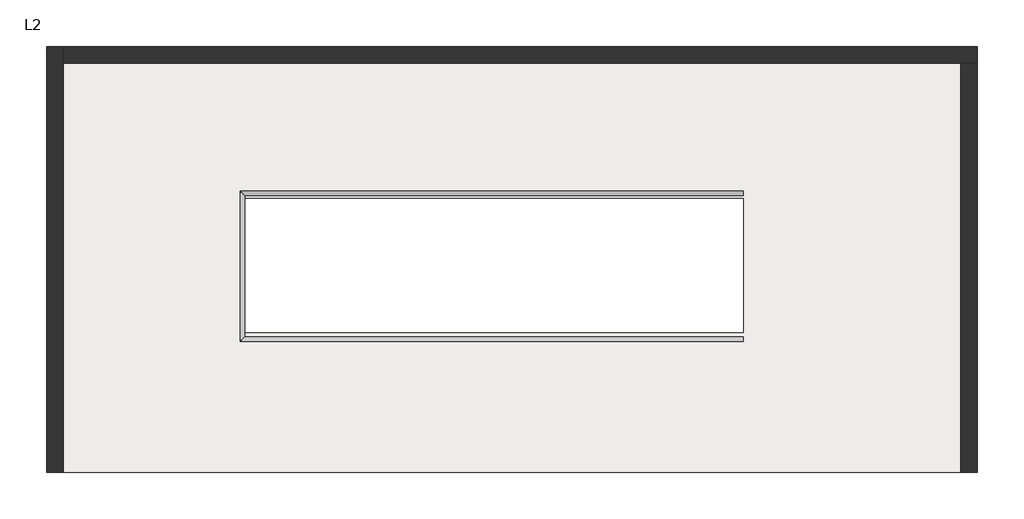
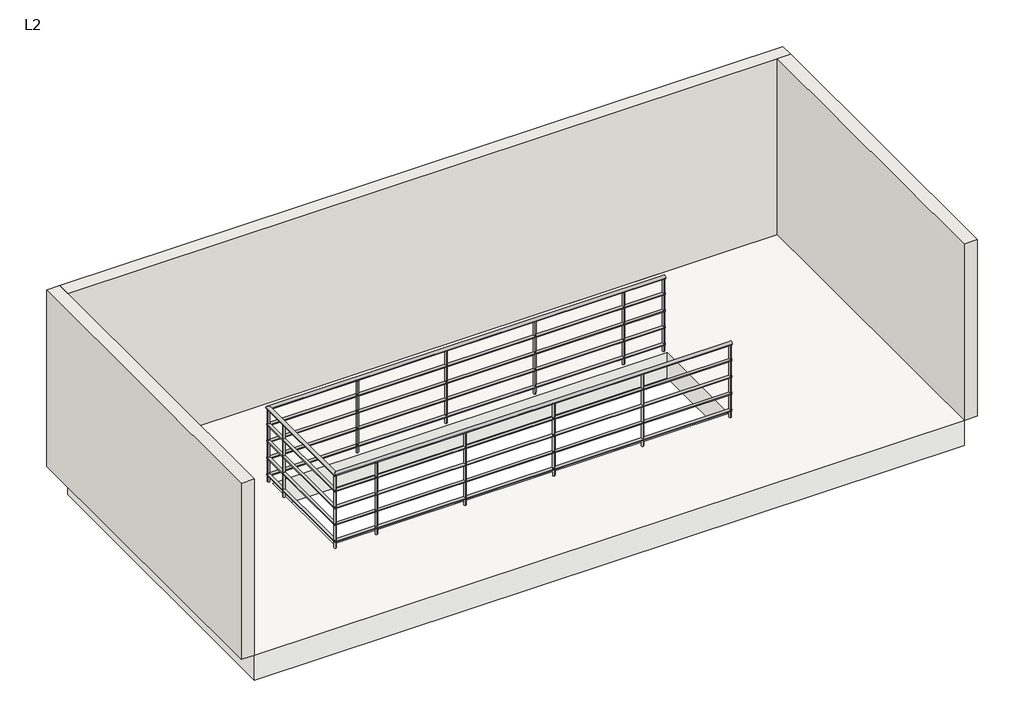
# One storey: 3 walls, 1 railing, 1 slab.
"""IFC4 building model written with IfcOpenShell, lengths in millimetres."""

from ifc_helpers import new_model, si_unit, point, frame, frame_2d, origin, place, context, project, spatial, polyline, circle_curve, ellipse_curve, trimmed, segment, composite_curve, outline, extrude, faceted_brep, element, save
from ifc_brep_helpers import plane_surface, cylinder_surface, advanced_brep

model = new_model("IFC4")

# Units and contexts
model_context = context("Model", 3, world=origin())
ifc_project = project(units=[si_unit("LENGTHUNIT", "METRE", prefix="MILLI")], contexts=[model_context])

# Site, building, storey
site = spatial("IfcSite", under=ifc_project)
building = spatial("IfcBuilding", under=site)
storey = spatial("IfcBuildingStorey", under=building, Name="L2", Elevation=2700.0)

# Railing
placement = place(None, origin())
element("IfcRailing", 1, ObjectType="900mm Pipe", at=placement, inside=storey, context=model_context, shape_type="SolidModel", body=[
    advanced_brep(
    [(-2164.8480531, 1633.4805305, 3580.0), (-2164.8480531, 1593.4805305, 3580.0), (-6608.8480531, 1633.4805305, 3580.0), (-6648.8480531, 1593.4805305, 3580.0), (-6608.8480531, 2893.4805305, 3580.0), (-6648.8480531, 2933.4805305, 3580.0), (-2164.8480531, 2893.4805305, 3580.0), (-2164.8480531, 2933.4805305, 3580.0)],
    [
        (0, 1, circle_curve(frame((-2164.8480531, 1613.4805305, 3580.0), z_axis=(1.0, 0.0, 0.0), x_axis=(0.0, -1.0, 0.0)), 20.0)),
        (1, 0, circle_curve(frame((-2164.8480531, 1613.4805305, 3580.0), z_axis=(1.0, 0.0, 0.0), x_axis=(0.0, -1.0, 0.0)), 20.0)),
        (0, 2),
        (2, 3, ellipse_curve(frame((-6628.8480531, 1613.4805305, 3580.0), z_axis=(0.7071067811865459, -0.7071067811865491, 0.0), x_axis=(0.7071067811865491, 0.7071067811865459, 0.0)), 28.2842712, 20.0)),
        (3, 1),
        (3, 2, ellipse_curve(frame((-6628.8480531, 1613.4805305, 3580.0), z_axis=(0.7071067811865459, -0.7071067811865491, 0.0), x_axis=(0.7071067811865491, 0.7071067811865459, 0.0)), 28.2842712, 20.0)),
        (2, 4),
        (4, 5, ellipse_curve(frame((-6628.8480531, 2913.4805305, 3580.0), z_axis=(-0.7071067811865492, -0.7071067811865458, 0.0), x_axis=(0.7071067811865457, -0.7071067811865493, 0.0)), 28.2842712, 20.0)),
        (5, 3),
        (5, 4, ellipse_curve(frame((-6628.8480531, 2913.4805305, 3580.0), z_axis=(-0.7071067811865492, -0.7071067811865458, 0.0), x_axis=(0.7071067811865457, -0.7071067811865493, 0.0)), 28.2842712, 20.0)),
        (6, 7, circle_curve(frame((-2164.8480531, 2913.4805305, 3580.0), z_axis=(1.0, 0.0, 0.0), x_axis=(0.0, 1.0, 0.0)), 20.0)),
        (7, 6, circle_curve(frame((-2164.8480531, 2913.4805305, 3580.0), z_axis=(1.0, 0.0, 0.0), x_axis=(0.0, 1.0, 0.0)), 20.0)),
        (4, 6),
        (7, 5),
    ],
    [
        plane_surface(frame((-2164.8480531, 1613.4805305, 3600.0), z_axis=(1.0, 0.0, 0.0), x_axis=(0.0, -1.0, 0.0))),
        cylinder_surface(frame((-2164.8480531, 1613.4805305, 3580.0), z_axis=(1.0, 0.0, 0.0), x_axis=(0.0, -1.0, 0.0)), 20.0),
        cylinder_surface(frame((-6628.8480531, 1613.4805305, 3580.0), z_axis=(0.0, -1.0, 0.0), x_axis=(-1.0, 0.0, 0.0)), 20.0),
        plane_surface(frame((-2164.8480531, 2913.4805305, 3600.0), z_axis=(1.0, 0.0, 0.0), x_axis=(0.0, 1.0, 0.0))),
        cylinder_surface(frame((-6628.8480531, 2913.4805305, 3580.0), z_axis=(-1.0, 0.0, 0.0), x_axis=(0.0, 1.0, 0.0)), 20.0),
    ],
    [
        (0, [[1, 2]]),
        (1, [[-1, 3, 4, 5]]),
        (1, [[-2, -5, 6, -3]]),
        (2, [[-4, 7, 8, 9]]),
        (2, [[-6, -9, 10, -7]]),
        (3, [[11, 12]]),
        (4, [[-8, 13, -12, 14]]),
        (4, [[-10, -14, -11, -13]]),
    ],
),
    advanced_brep(
    [(-2164.8480531, 1598.4805305, 3385.0), (-2164.8480531, 1628.4805305, 3385.0), (-6643.8480531, 1598.4805305, 3385.0), (-6613.8480531, 1628.4805305, 3385.0), (-6643.8480531, 2928.4805305, 3385.0), (-6613.8480531, 2898.4805305, 3385.0), (-2164.8480531, 2928.4805305, 3385.0), (-2164.8480531, 2898.4805305, 3385.0)],
    [
        (0, 1, circle_curve(frame((-2164.8480531, 1613.4805305, 3385.0), z_axis=(1.0, 0.0, 0.0), x_axis=(0.0, 1.0, 0.0)), 15.0)),
        (1, 0, circle_curve(frame((-2164.8480531, 1613.4805305, 3385.0), z_axis=(1.0, 0.0, 0.0), x_axis=(0.0, 1.0, 0.0)), 15.0)),
        (0, 2),
        (2, 3, ellipse_curve(frame((-6628.8480531, 1613.4805305, 3385.0), z_axis=(0.7071067811865459, -0.7071067811865491, 0.0), x_axis=(0.7071067811865491, 0.7071067811865459, 0.0)), 21.2132034, 15.0)),
        (3, 1),
        (3, 2, ellipse_curve(frame((-6628.8480531, 1613.4805305, 3385.0), z_axis=(0.7071067811865459, -0.7071067811865491, 0.0), x_axis=(0.7071067811865491, 0.7071067811865459, 0.0)), 21.2132034, 15.0)),
        (2, 4),
        (4, 5, ellipse_curve(frame((-6628.8480531, 2913.4805305, 3385.0), z_axis=(-0.7071067811865492, -0.7071067811865458, 0.0), x_axis=(0.7071067811865457, -0.7071067811865493, 0.0)), 21.2132034, 15.0)),
        (5, 3),
        (5, 4, ellipse_curve(frame((-6628.8480531, 2913.4805305, 3385.0), z_axis=(-0.7071067811865492, -0.7071067811865458, 0.0), x_axis=(0.7071067811865457, -0.7071067811865493, 0.0)), 21.2132034, 15.0)),
        (6, 7, circle_curve(frame((-2164.8480531, 2913.4805305, 3385.0), z_axis=(1.0, 0.0, 0.0), x_axis=(0.0, -1.0, 0.0)), 15.0)),
        (7, 6, circle_curve(frame((-2164.8480531, 2913.4805305, 3385.0), z_axis=(1.0, 0.0, 0.0), x_axis=(0.0, -1.0, 0.0)), 15.0)),
        (4, 6),
        (7, 5),
    ],
    [
        plane_surface(frame((-2164.8480531, 1613.4805305, 3400.0), z_axis=(1.0, 0.0, 0.0), x_axis=(0.0, -1.0, 0.0))),
        cylinder_surface(frame((-2164.8480531, 1613.4805305, 3385.0), z_axis=(1.0, 0.0, 0.0), x_axis=(0.0, 1.0, 0.0)), 15.0),
        cylinder_surface(frame((-6628.8480531, 1613.4805305, 3385.0), z_axis=(0.0, -1.0, 0.0), x_axis=(1.0, 0.0, 0.0)), 15.0),
        plane_surface(frame((-2164.8480531, 2913.4805305, 3400.0), z_axis=(1.0, 0.0, 0.0), x_axis=(0.0, 1.0, 0.0))),
        cylinder_surface(frame((-6628.8480531, 2913.4805305, 3385.0), z_axis=(-1.0, 0.0, 0.0), x_axis=(0.0, -1.0, 0.0)), 15.0),
    ],
    [
        (0, [[1, 2]]),
        (1, [[-1, 3, 4, 5]]),
        (1, [[-2, -5, 6, -3]]),
        (2, [[-4, 7, 8, 9]]),
        (2, [[-6, -9, 10, -7]]),
        (3, [[11, 12]]),
        (4, [[-8, 13, -12, 14]]),
        (4, [[-10, -14, -11, -13]]),
    ],
),
    advanced_brep(
    [(-2164.8480531, 1598.4805305, 3185.0), (-2164.8480531, 1628.4805305, 3185.0), (-6643.8480531, 1598.4805305, 3185.0), (-6613.8480531, 1628.4805305, 3185.0), (-6643.8480531, 2928.4805305, 3185.0), (-6613.8480531, 2898.4805305, 3185.0), (-2164.8480531, 2928.4805305, 3185.0), (-2164.8480531, 2898.4805305, 3185.0)],
    [
        (0, 1, circle_curve(frame((-2164.8480531, 1613.4805305, 3185.0), z_axis=(1.0, 0.0, 0.0), x_axis=(0.0, 1.0, 0.0)), 15.0)),
        (1, 0, circle_curve(frame((-2164.8480531, 1613.4805305, 3185.0), z_axis=(1.0, 0.0, 0.0), x_axis=(0.0, 1.0, 0.0)), 15.0)),
        (0, 2),
        (2, 3, ellipse_curve(frame((-6628.8480531, 1613.4805305, 3185.0), z_axis=(0.7071067811865459, -0.7071067811865491, 0.0), x_axis=(0.7071067811865491, 0.7071067811865459, 0.0)), 21.2132034, 15.0)),
        (3, 1),
        (3, 2, ellipse_curve(frame((-6628.8480531, 1613.4805305, 3185.0), z_axis=(0.7071067811865459, -0.7071067811865491, 0.0), x_axis=(0.7071067811865491, 0.7071067811865459, 0.0)), 21.2132034, 15.0)),
        (2, 4),
        (4, 5, ellipse_curve(frame((-6628.8480531, 2913.4805305, 3185.0), z_axis=(-0.7071067811865492, -0.7071067811865458, 0.0), x_axis=(0.7071067811865457, -0.7071067811865493, 0.0)), 21.2132034, 15.0)),
        (5, 3),
        (5, 4, ellipse_curve(frame((-6628.8480531, 2913.4805305, 3185.0), z_axis=(-0.7071067811865492, -0.7071067811865458, 0.0), x_axis=(0.7071067811865457, -0.7071067811865493, 0.0)), 21.2132034, 15.0)),
        (6, 7, circle_curve(frame((-2164.8480531, 2913.4805305, 3185.0), z_axis=(1.0, 0.0, 0.0), x_axis=(0.0, -1.0, 0.0)), 15.0)),
        (7, 6, circle_curve(frame((-2164.8480531, 2913.4805305, 3185.0), z_axis=(1.0, 0.0, 0.0), x_axis=(0.0, -1.0, 0.0)), 15.0)),
        (4, 6),
        (7, 5),
    ],
    [
        plane_surface(frame((-2164.8480531, 1613.4805305, 3200.0), z_axis=(1.0, 0.0, 0.0), x_axis=(0.0, -1.0, 0.0))),
        cylinder_surface(frame((-2164.8480531, 1613.4805305, 3185.0), z_axis=(1.0, 0.0, 0.0), x_axis=(0.0, 1.0, 0.0)), 15.0),
        cylinder_surface(frame((-6628.8480531, 1613.4805305, 3185.0), z_axis=(0.0, -1.0, 0.0), x_axis=(1.0, 0.0, 0.0)), 15.0),
        plane_surface(frame((-2164.8480531, 2913.4805305, 3200.0), z_axis=(1.0, 0.0, 0.0), x_axis=(0.0, 1.0, 0.0))),
        cylinder_surface(frame((-6628.8480531, 2913.4805305, 3185.0), z_axis=(-1.0, 0.0, 0.0), x_axis=(0.0, -1.0, 0.0)), 15.0),
    ],
    [
        (0, [[1, 2]]),
        (1, [[-1, 3, 4, 5]]),
        (1, [[-2, -5, 6, -3]]),
        (2, [[-4, 7, 8, 9]]),
        (2, [[-6, -9, 10, -7]]),
        (3, [[11, 12]]),
        (4, [[-8, 13, -12, 14]]),
        (4, [[-10, -14, -11, -13]]),
    ],
),
    advanced_brep(
    [(-2164.8480531, 1598.4805305, 2985.0), (-2164.8480531, 1628.4805305, 2985.0), (-6643.8480531, 1598.4805305, 2985.0), (-6613.8480531, 1628.4805305, 2985.0), (-6643.8480531, 2928.4805305, 2985.0), (-6613.8480531, 2898.4805305, 2985.0), (-2164.8480531, 2928.4805305, 2985.0), (-2164.8480531, 2898.4805305, 2985.0)],
    [
        (0, 1, circle_curve(frame((-2164.8480531, 1613.4805305, 2985.0), z_axis=(1.0, 0.0, 0.0), x_axis=(0.0, 1.0, 0.0)), 15.0)),
        (1, 0, circle_curve(frame((-2164.8480531, 1613.4805305, 2985.0), z_axis=(1.0, 0.0, 0.0), x_axis=(0.0, 1.0, 0.0)), 15.0)),
        (0, 2),
        (2, 3, ellipse_curve(frame((-6628.8480531, 1613.4805305, 2985.0), z_axis=(0.7071067811865459, -0.7071067811865491, 0.0), x_axis=(0.7071067811865491, 0.7071067811865459, 0.0)), 21.2132034, 15.0)),
        (3, 1),
        (3, 2, ellipse_curve(frame((-6628.8480531, 1613.4805305, 2985.0), z_axis=(0.7071067811865459, -0.7071067811865491, 0.0), x_axis=(0.7071067811865491, 0.7071067811865459, 0.0)), 21.2132034, 15.0)),
        (2, 4),
        (4, 5, ellipse_curve(frame((-6628.8480531, 2913.4805305, 2985.0), z_axis=(-0.7071067811865492, -0.7071067811865458, 0.0), x_axis=(0.7071067811865457, -0.7071067811865493, 0.0)), 21.2132034, 15.0)),
        (5, 3),
        (5, 4, ellipse_curve(frame((-6628.8480531, 2913.4805305, 2985.0), z_axis=(-0.7071067811865492, -0.7071067811865458, 0.0), x_axis=(0.7071067811865457, -0.7071067811865493, 0.0)), 21.2132034, 15.0)),
        (6, 7, circle_curve(frame((-2164.8480531, 2913.4805305, 2985.0), z_axis=(1.0, 0.0, 0.0), x_axis=(0.0, -1.0, 0.0)), 15.0)),
        (7, 6, circle_curve(frame((-2164.8480531, 2913.4805305, 2985.0), z_axis=(1.0, 0.0, 0.0), x_axis=(0.0, -1.0, 0.0)), 15.0)),
        (4, 6),
        (7, 5),
    ],
    [
        plane_surface(frame((-2164.8480531, 1613.4805305, 3000.0), z_axis=(1.0, 0.0, 0.0), x_axis=(0.0, -1.0, 0.0))),
        cylinder_surface(frame((-2164.8480531, 1613.4805305, 2985.0), z_axis=(1.0, 0.0, 0.0), x_axis=(0.0, 1.0, 0.0)), 15.0),
        cylinder_surface(frame((-6628.8480531, 1613.4805305, 2985.0), z_axis=(0.0, -1.0, 0.0), x_axis=(1.0, 0.0, 0.0)), 15.0),
        plane_surface(frame((-2164.8480531, 2913.4805305, 3000.0), z_axis=(1.0, 0.0, 0.0), x_axis=(0.0, 1.0, 0.0))),
        cylinder_surface(frame((-6628.8480531, 2913.4805305, 2985.0), z_axis=(-1.0, 0.0, 0.0), x_axis=(0.0, -1.0, 0.0)), 15.0),
    ],
    [
        (0, [[1, 2]]),
        (1, [[-1, 3, 4, 5]]),
        (1, [[-2, -5, 6, -3]]),
        (2, [[-4, 7, 8, 9]]),
        (2, [[-6, -9, 10, -7]]),
        (3, [[11, 12]]),
        (4, [[-8, 13, -12, 14]]),
        (4, [[-10, -14, -11, -13]]),
    ],
),
    advanced_brep(
    [(-2164.8480531, 1598.4805305, 2785.0), (-2164.8480531, 1628.4805305, 2785.0), (-6643.8480531, 1598.4805305, 2785.0), (-6613.8480531, 1628.4805305, 2785.0), (-6643.8480531, 2928.4805305, 2785.0), (-6613.8480531, 2898.4805305, 2785.0), (-2164.8480531, 2928.4805305, 2785.0), (-2164.8480531, 2898.4805305, 2785.0)],
    [
        (0, 1, circle_curve(frame((-2164.8480531, 1613.4805305, 2785.0), z_axis=(1.0, 0.0, 0.0), x_axis=(0.0, 1.0, 0.0)), 15.0)),
        (1, 0, circle_curve(frame((-2164.8480531, 1613.4805305, 2785.0), z_axis=(1.0, 0.0, 0.0), x_axis=(0.0, 1.0, 0.0)), 15.0)),
        (0, 2),
        (2, 3, ellipse_curve(frame((-6628.8480531, 1613.4805305, 2785.0), z_axis=(0.7071067811865459, -0.7071067811865491, 0.0), x_axis=(0.7071067811865491, 0.7071067811865459, 0.0)), 21.2132034, 15.0)),
        (3, 1),
        (3, 2, ellipse_curve(frame((-6628.8480531, 1613.4805305, 2785.0), z_axis=(0.7071067811865459, -0.7071067811865491, 0.0), x_axis=(0.7071067811865491, 0.7071067811865459, 0.0)), 21.2132034, 15.0)),
        (2, 4),
        (4, 5, ellipse_curve(frame((-6628.8480531, 2913.4805305, 2785.0), z_axis=(-0.7071067811865492, -0.7071067811865458, 0.0), x_axis=(0.7071067811865457, -0.7071067811865493, 0.0)), 21.2132034, 15.0)),
        (5, 3),
        (5, 4, ellipse_curve(frame((-6628.8480531, 2913.4805305, 2785.0), z_axis=(-0.7071067811865492, -0.7071067811865458, 0.0), x_axis=(0.7071067811865457, -0.7071067811865493, 0.0)), 21.2132034, 15.0)),
        (6, 7, circle_curve(frame((-2164.8480531, 2913.4805305, 2785.0), z_axis=(1.0, 0.0, 0.0), x_axis=(0.0, -1.0, 0.0)), 15.0)),
        (7, 6, circle_curve(frame((-2164.8480531, 2913.4805305, 2785.0), z_axis=(1.0, 0.0, 0.0), x_axis=(0.0, -1.0, 0.0)), 15.0)),
        (4, 6),
        (7, 5),
    ],
    [
        plane_surface(frame((-2164.8480531, 1613.4805305, 2800.0), z_axis=(1.0, 0.0, 0.0), x_axis=(0.0, -1.0, 0.0))),
        cylinder_surface(frame((-2164.8480531, 1613.4805305, 2785.0), z_axis=(1.0, 0.0, 0.0), x_axis=(0.0, 1.0, 0.0)), 15.0),
        cylinder_surface(frame((-6628.8480531, 1613.4805305, 2785.0), z_axis=(0.0, -1.0, 0.0), x_axis=(1.0, 0.0, 0.0)), 15.0),
        plane_surface(frame((-2164.8480531, 2913.4805305, 2800.0), z_axis=(1.0, 0.0, 0.0), x_axis=(0.0, 1.0, 0.0))),
        cylinder_surface(frame((-6628.8480531, 2913.4805305, 2785.0), z_axis=(-1.0, 0.0, 0.0), x_axis=(0.0, -1.0, 0.0)), 15.0),
    ],
    [
        (0, [[1, 2]]),
        (1, [[-1, 3, 4, 5]]),
        (1, [[-2, -5, 6, -3]]),
        (2, [[-4, 7, 8, 9]]),
        (2, [[-6, -9, 10, -7]]),
        (3, [[11, 12]]),
        (4, [[-8, 13, -12, 14]]),
        (4, [[-10, -14, -11, -13]]),
    ],
),
    extrude(outline(composite_curve([segment(trimmed(circle_curve(frame_2d((-2628.8480531, 2913.4805305)), 12.5), [point((-2628.8480531, 2925.9805305))], [point((-2628.8480531, 2900.9805305))], False, "CARTESIAN"), True, "CONTINUOUS"), segment(trimmed(circle_curve(frame_2d((-2628.8480531, 2913.4805305)), 12.5), [point((-2628.8480531, 2900.9805305))], [point((-2628.8480531, 2925.9805305))], False, "CARTESIAN"), True, "CONTINUOUS")], self_intersect=False)), frame((0.0, 0.0, 2700.0), z_axis=(0.0, 0.0, 1.0), x_axis=(1.0, 0.0, 0.0)), (0.0, 0.0, 1.0), 860.0),
    extrude(outline(composite_curve([segment(trimmed(circle_curve(frame_2d((-3628.8480531, 2913.4805305)), 12.5), [point((-3628.8480531, 2925.9805305))], [point((-3628.8480531, 2900.9805305))], False, "CARTESIAN"), True, "CONTINUOUS"), segment(trimmed(circle_curve(frame_2d((-3628.8480531, 2913.4805305)), 12.5), [point((-3628.8480531, 2900.9805305))], [point((-3628.8480531, 2925.9805305))], False, "CARTESIAN"), True, "CONTINUOUS")], self_intersect=False)), frame((0.0, 0.0, 2700.0), z_axis=(0.0, 0.0, 1.0), x_axis=(1.0, 0.0, 0.0)), (0.0, 0.0, 1.0), 860.0),
    extrude(outline(composite_curve([segment(trimmed(circle_curve(frame_2d((-4628.8480531, 2913.4805305)), 12.5), [point((-4628.8480531, 2925.9805305))], [point((-4628.8480531, 2900.9805305))], False, "CARTESIAN"), True, "CONTINUOUS"), segment(trimmed(circle_curve(frame_2d((-4628.8480531, 2913.4805305)), 12.5), [point((-4628.8480531, 2900.9805305))], [point((-4628.8480531, 2925.9805305))], False, "CARTESIAN"), True, "CONTINUOUS")], self_intersect=False)), frame((0.0, 0.0, 2700.0), z_axis=(0.0, 0.0, 1.0), x_axis=(1.0, 0.0, 0.0)), (0.0, 0.0, 1.0), 860.0),
    extrude(outline(composite_curve([segment(trimmed(circle_curve(frame_2d((-5628.8480531, 2913.4805305)), 12.5), [point((-5628.8480531, 2925.9805305))], [point((-5628.8480531, 2900.9805305))], False, "CARTESIAN"), True, "CONTINUOUS"), segment(trimmed(circle_curve(frame_2d((-5628.8480531, 2913.4805305)), 12.5), [point((-5628.8480531, 2900.9805305))], [point((-5628.8480531, 2925.9805305))], False, "CARTESIAN"), True, "CONTINUOUS")], self_intersect=False)), frame((0.0, 0.0, 2700.0), z_axis=(0.0, 0.0, 1.0), x_axis=(1.0, 0.0, 0.0)), (0.0, 0.0, 1.0), 860.0),
    extrude(outline(composite_curve([segment(trimmed(circle_curve(frame_2d((-6628.8480531, 2613.4805305)), 12.5), [point((-6641.3480531, 2613.4805305))], [point((-6616.3480531, 2613.4805305))], False, "CARTESIAN"), True, "CONTINUOUS"), segment(trimmed(circle_curve(frame_2d((-6628.8480531, 2613.4805305)), 12.5), [point((-6616.3480531, 2613.4805305))], [point((-6641.3480531, 2613.4805305))], False, "CARTESIAN"), True, "CONTINUOUS")], self_intersect=False)), frame((0.0, 0.0, 2700.0), z_axis=(0.0, 0.0, 1.0), x_axis=(1.0, 0.0, 0.0)), (0.0, 0.0, 1.0), 860.0),
    extrude(outline(composite_curve([segment(trimmed(circle_curve(frame_2d((-6164.8480531, 1613.4805305)), 12.5), [point((-6164.8480531, 1600.9805305))], [point((-6164.8480531, 1625.9805305))], False, "CARTESIAN"), True, "CONTINUOUS"), segment(trimmed(circle_curve(frame_2d((-6164.8480531, 1613.4805305)), 12.5), [point((-6164.8480531, 1625.9805305))], [point((-6164.8480531, 1600.9805305))], False, "CARTESIAN"), True, "CONTINUOUS")], self_intersect=False)), frame((0.0, 0.0, 2700.0), z_axis=(0.0, 0.0, 1.0), x_axis=(1.0, 0.0, 0.0)), (0.0, 0.0, 1.0), 860.0),
    extrude(outline(composite_curve([segment(trimmed(circle_curve(frame_2d((-5164.8480531, 1613.4805305)), 12.5), [point((-5164.8480531, 1600.9805305))], [point((-5164.8480531, 1625.9805305))], False, "CARTESIAN"), True, "CONTINUOUS"), segment(trimmed(circle_curve(frame_2d((-5164.8480531, 1613.4805305)), 12.5), [point((-5164.8480531, 1625.9805305))], [point((-5164.8480531, 1600.9805305))], False, "CARTESIAN"), True, "CONTINUOUS")], self_intersect=False)), frame((0.0, 0.0, 2700.0), z_axis=(0.0, 0.0, 1.0), x_axis=(1.0, 0.0, 0.0)), (0.0, 0.0, 1.0), 860.0),
    extrude(outline(composite_curve([segment(trimmed(circle_curve(frame_2d((-4164.8480531, 1613.4805305)), 12.5), [point((-4164.8480531, 1600.9805305))], [point((-4164.8480531, 1625.9805305))], False, "CARTESIAN"), True, "CONTINUOUS"), segment(trimmed(circle_curve(frame_2d((-4164.8480531, 1613.4805305)), 12.5), [point((-4164.8480531, 1625.9805305))], [point((-4164.8480531, 1600.9805305))], False, "CARTESIAN"), True, "CONTINUOUS")], self_intersect=False)), frame((0.0, 0.0, 2700.0), z_axis=(0.0, 0.0, 1.0), x_axis=(1.0, 0.0, 0.0)), (0.0, 0.0, 1.0), 860.0),
    extrude(outline(composite_curve([segment(trimmed(circle_curve(frame_2d((-3164.8480531, 1613.4805305)), 12.5), [point((-3164.8480531, 1600.9805305))], [point((-3164.8480531, 1625.9805305))], False, "CARTESIAN"), True, "CONTINUOUS"), segment(trimmed(circle_curve(frame_2d((-3164.8480531, 1613.4805305)), 12.5), [point((-3164.8480531, 1625.9805305))], [point((-3164.8480531, 1600.9805305))], False, "CARTESIAN"), True, "CONTINUOUS")], self_intersect=False)), frame((0.0, 0.0, 2700.0), z_axis=(0.0, 0.0, 1.0), x_axis=(1.0, 0.0, 0.0)), (0.0, 0.0, 1.0), 860.0),
    extrude(outline(composite_curve([segment(trimmed(circle_curve(frame_2d((-6628.8480531, 2913.4805305)), 12.5), [point((-6641.3480531, 2913.4805305))], [point((-6616.3480531, 2913.4805305))], False, "CARTESIAN"), True, "CONTINUOUS"), segment(trimmed(circle_curve(frame_2d((-6628.8480531, 2913.4805305)), 12.5), [point((-6616.3480531, 2913.4805305))], [point((-6641.3480531, 2913.4805305))], False, "CARTESIAN"), True, "CONTINUOUS")], self_intersect=False)), frame((0.0, 0.0, 2700.0), z_axis=(0.0, 0.0, 1.0), x_axis=(1.0, 0.0, 0.0)), (0.0, 0.0, 1.0), 860.0),
    extrude(outline(composite_curve([segment(trimmed(circle_curve(frame_2d((-6628.8480531, 1613.4805305)), 12.5), [point((-6628.8480531, 1600.9805305))], [point((-6628.8480531, 1625.9805305))], False, "CARTESIAN"), True, "CONTINUOUS"), segment(trimmed(circle_curve(frame_2d((-6628.8480531, 1613.4805305)), 12.5), [point((-6628.8480531, 1625.9805305))], [point((-6628.8480531, 1600.9805305))], False, "CARTESIAN"), True, "CONTINUOUS")], self_intersect=False)), frame((0.0, 0.0, 2700.0), z_axis=(0.0, 0.0, 1.0), x_axis=(1.0, 0.0, 0.0)), (0.0, 0.0, 1.0), 860.0),
    extrude(outline(composite_curve([segment(trimmed(circle_curve(frame_2d((-2177.3480531, 2913.4805305)), 12.5), [point((-2177.3480531, 2925.9805305))], [point((-2177.3480531, 2900.9805305))], False, "CARTESIAN"), True, "CONTINUOUS"), segment(trimmed(circle_curve(frame_2d((-2177.3480531, 2913.4805305)), 12.5), [point((-2177.3480531, 2900.9805305))], [point((-2177.3480531, 2925.9805305))], False, "CARTESIAN"), True, "CONTINUOUS")], self_intersect=False)), frame((0.0, 0.0, 2700.0), z_axis=(0.0, 0.0, 1.0), x_axis=(1.0, 0.0, 0.0)), (0.0, 0.0, 1.0), 860.0),
    extrude(outline(composite_curve([segment(trimmed(circle_curve(frame_2d((-2177.3480531, 1613.4805305)), 12.5), [point((-2177.3480531, 1600.9805305))], [point((-2177.3480531, 1625.9805305))], False, "CARTESIAN"), True, "CONTINUOUS"), segment(trimmed(circle_curve(frame_2d((-2177.3480531, 1613.4805305)), 12.5), [point((-2177.3480531, 1625.9805305))], [point((-2177.3480531, 1600.9805305))], False, "CARTESIAN"), True, "CONTINUOUS")], self_intersect=False)), frame((0.0, 0.0, 2700.0), z_axis=(0.0, 0.0, 1.0), x_axis=(1.0, 0.0, 0.0)), (0.0, 0.0, 1.0), 860.0),
])

# Slab
element("IfcSlab", 2, ObjectType="Generic 300mm", at=placement, inside=storey, context=model_context, shape_type="SweptSolid", body=[
    extrude(outline(polyline([(-8225.0, 4075.0), (-5925.0, 4075.0), (-1461.0, 4075.0), (-225.0, 4075.0), (-225.0, 425.0), (-8225.0, 425.0), (-8225.0, 4075.0)]), holes=[polyline([(-2161.0, 2869.6), (-6608.8480531, 2869.6), (-6608.8480531, 1675.0), (-2161.0, 1675.0), (-2161.0, 2869.6)])]), frame((0.0, 0.0, 2400.0), z_axis=(0.0, 0.0, 1.0), x_axis=(1.0, 0.0, 0.0)), (0.0, 0.0, 1.0), 300.0),
])

# Walls
element("IfcWall", 3, ObjectType="Generic - 150mm", at=placement, inside=storey, context=model_context, shape_type="Brep", body=[
    faceted_brep([(-8225.0, 425.0, 2700.0), (-8225.0, 4075.0, 2700.0), (-8225.0, 4225.0, 2700.0), (-8225.0, 4225.0, 4800.0), (-8225.0, 4075.0, 4800.0), (-8225.0, 425.0, 4800.0), (-8375.0, 425.0, 2700.0), (-8375.0, 425.0, 4800.0), (-8375.0, 4225.0, 4800.0), (-8375.0, 4225.0, 2700.0)], [[[0, 1, 2, 3, 4, 5]], [[6, 7, 8, 9]], [[2, 1, 0, 6, 9]], [[5, 4, 3, 8, 7]], [[0, 5, 7, 6]], [[3, 2, 9, 8]]]),
])
element("IfcWall", 4, ObjectType="Generic - 150mm", at=placement, inside=storey, context=model_context, shape_type="Brep", body=[
    faceted_brep([(-8225.0, 4075.0, 2700.0), (-225.0, 4075.0, 2700.0), (-75.0, 4075.0, 2700.0), (-75.0, 4075.0, 4800.0), (-225.0, 4075.0, 4800.0), (-8225.0, 4075.0, 4800.0), (-8225.0, 4225.0, 2700.0), (-8225.0, 4225.0, 4800.0), (-75.0, 4225.0, 4800.0), (-75.0, 4225.0, 2700.0)], [[[0, 1, 2, 3, 4, 5]], [[6, 7, 8, 9]], [[2, 1, 0, 6, 9]], [[5, 4, 3, 8, 7]], [[0, 5, 7, 6]], [[3, 2, 9, 8]]]),
])
element("IfcWall", 5, ObjectType="Generic - 150mm", at=placement, inside=storey, context=model_context, shape_type="SweptSolid", body=[
    extrude(outline(polyline([(-225.0, 425.0), (-225.0, 4075.0), (-75.0, 4075.0), (-75.0, 425.0), (-225.0, 425.0)])), frame((0.0, 0.0, 2700.0), z_axis=(0.0, 0.0, 1.0), x_axis=(1.0, 0.0, 0.0)), (0.0, 0.0, 1.0), 2100.0),
])

save(model, "model.ifc")

# Revit data of these elements
# Type "900mm Pipe"
#   built-in parameter 1008612 = 0.019685 (stored number, unit not read)
#   built-in parameter 1008611 = 0.0984252 (stored number, unit not read)
#   built-in parameter 1008609 = 3.28084 (stored number, unit not read)
#   built-in parameter 1008604 = 0.19685 (stored number, unit not read)
#   built-in parameter 1008603 = 0.164042 (stored number, unit not read)
#   Railing Height = 900 mm
#   built-in parameter 1008630 = 2
#   built-in parameter 1008610 = 1
#   built-in parameter 1008605 = 1
#   built-in parameter 1008618 = M_Baluster - Round : 25mm
# Type "Generic 300mm"
#   Description = "Generic Floor (Material By Category), 300mm thick"
#   Function = 0
#   Layers, outside or top first: 300 mm no material (function 1)
# Type "Generic - 150mm"
#   Description = "Generic Wall (Material By Category), 150mm thick"
#   Type Mark = "G04"
#   Layers, outside or top first: 150 mm no material (function 1)
# Element 1 (IfcRailing, "900mm Pipe")
#   Phase Created = New Construction
# Element 2 (IfcSlab, "Generic 300mm")
#   Height Offset From Level = 0 mm
#   Phase Created = New Construction
#   Materials on its faces: "Default Floor"
# Elements 3, 4, 5 (IfcWall, "Generic - 150mm")
#   Top Offset = 0 mm
#   Base Offset = 0 mm
#   Unconnected Height = 2100 mm
#   wall height = 2100 mm
#   Phase Created = New Construction
#   Base Constraint = L2
#   Materials on its faces: "Default Wall"
# Materials
#   "Default Floor": class "Miscellaneous", colour RGB 128 128 128, transparency 0, Cost = 0
#   "Default Wall": class "Miscellaneous", colour RGB 192 192 192, transparency 0, Cost = 0
